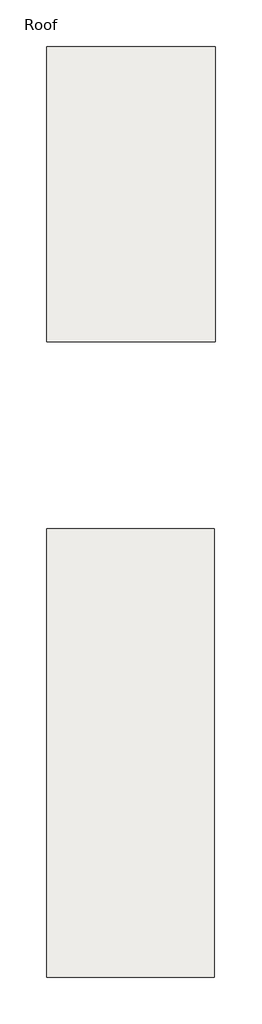
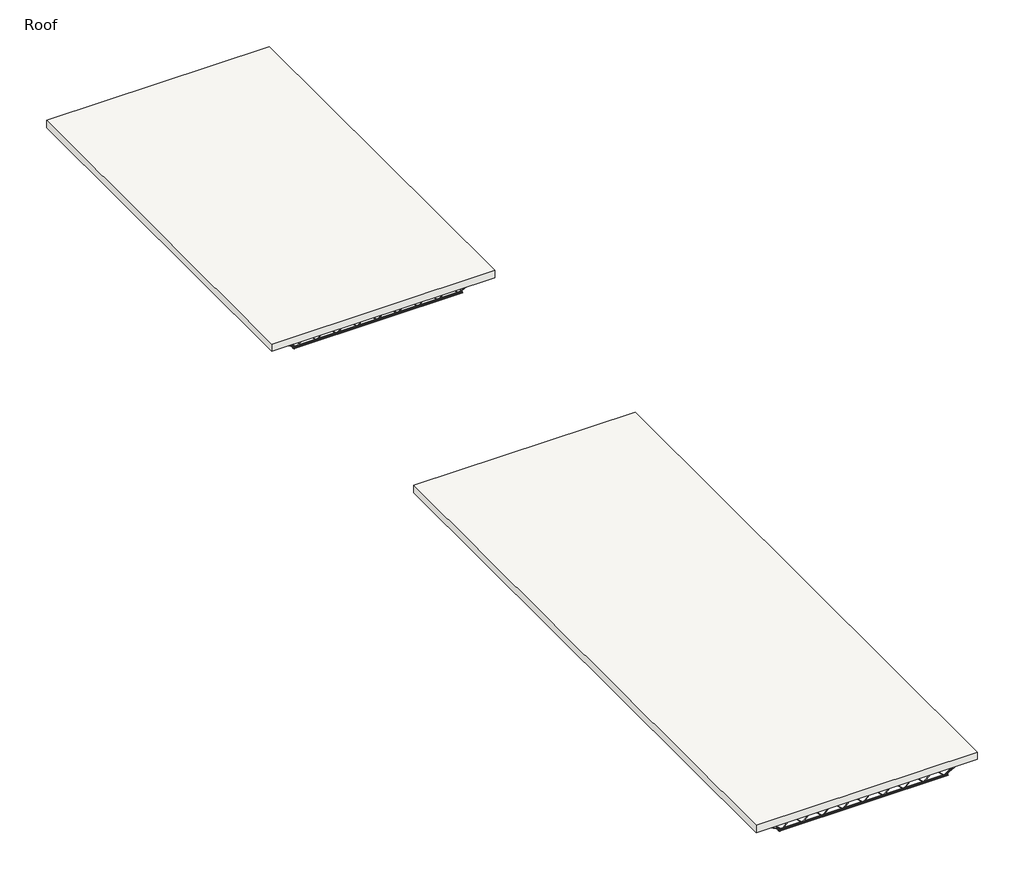
# One storey: 15 beams, 2 roofs.
"""IFC4 building model written with IfcOpenShell, lengths in millimetres."""

import ifcopenshell
import ifcopenshell.guid

model = None  # the IFC model being written
_history = None  # IfcOwnerHistory: only IFC2X3 demands one
_inside = {}  # id of a spatial element -> (the spatial element, [elements in it])
_under = {}  # id of a project, library or spatial element -> (it, [spatial elements below it])
_declared = {}  # id of a project -> (the project, [libraries it declares])
_typed = {}  # id of a type object -> (the type object, [elements of that type])
_made_of = {}  # id of a material, layer set ... -> (it, [elements and type objects made of it])


def new_model(schema):
    """Start an empty IFC model of exactly this schema.

    Asked for "IFC4X3", IfcOpenShell would pick the latest addendum, in which some entities
    have other attributes; the version numbers below select the first issue.
    IFC2X3 requires an IfcOwnerHistory on every rooted entity: one is made here for all.
    """
    global model, _history
    if schema == "IFC4X3":
        model = ifcopenshell.file(schema_version=(4, 3, 0, 0))
    else:
        model = ifcopenshell.file(schema=schema)
    _inside.clear()
    _under.clear()
    _declared.clear()
    _typed.clear()
    _made_of.clear()
    _history = None
    if model.schema == "IFC2X3":
        org = make("IfcOrganization", Name="unknown")
        user = make(
            "IfcPersonAndOrganization",
            ThePerson=make("IfcPerson", FamilyName="unknown"),
            TheOrganization=org,
        )
        app = make(
            "IfcApplication",
            ApplicationDeveloper=org,
            Version="unknown",
            ApplicationFullName="unknown",
            ApplicationIdentifier="unknown",
        )
        _history = make(
            "IfcOwnerHistory",
            OwningUser=user,
            OwningApplication=app,
            ChangeAction="ADDED",
            CreationDate=0,
        )
    return model


def make(cls, **values):
    """One entity of the class cls with the attributes given. An attribute that is None is left unset."""
    return model.create_entity(
        cls, **{name: value for name, value in values.items() if value is not None}
    )


def rooted(cls, **values):
    """An entity with a GlobalId (a new one), such as an element, a storey or a relation."""
    return make(cls, GlobalId=ifcopenshell.guid.new(), OwnerHistory=_history, **values)


def si_unit(unit_type, name, prefix=None):
    """IfcSIUnit, for example si_unit("LENGTHUNIT", "METRE", prefix="MILLI")."""
    return make("IfcSIUnit", UnitType=unit_type, Prefix=prefix, Name=name)


def assignment(units):
    """IfcUnitAssignment: the units of a project."""
    return None if units is None else make("IfcUnitAssignment", Units=units)


def point(xyz):
    """IfcCartesianPoint."""
    return None if xyz is None else make("IfcCartesianPoint", Coordinates=xyz)


def direction(xyz):
    """IfcDirection."""
    return None if xyz is None else make("IfcDirection", DirectionRatios=xyz)


def frame(location, z_axis=None, x_axis=None):
    """IfcAxis2Placement3D, a coordinate frame: its origin and axes. An axis left out is left unset."""
    return make(
        "IfcAxis2Placement3D",
        Location=point(location),
        Axis=direction(z_axis),
        RefDirection=direction(x_axis),
    )


def origin():
    """The frame at (0, 0, 0) with its axes left unset."""
    return frame((0.0, 0.0, 0.0))


def place(relative_to, where):
    """IfcLocalPlacement: puts the frame where relative to a parent placement (None: the world)."""
    return make(
        "IfcLocalPlacement", PlacementRelTo=relative_to, RelativePlacement=where
    )


def context(
    kind, dimensions, precision=None, world=None, true_north=None, identifier=None
):
    """IfcGeometricRepresentationContext, for example the 3D "Model" context."""
    return make(
        "IfcGeometricRepresentationContext",
        ContextIdentifier=identifier,
        ContextType=kind,
        CoordinateSpaceDimension=dimensions,
        Precision=precision,
        WorldCoordinateSystem=world,
        TrueNorth=true_north,
    )


def project(units=None, contexts=None):
    """IfcProject with its units and contexts."""
    return rooted(
        "IfcProject",
        Name="project",
        RepresentationContexts=contexts,
        UnitsInContext=assignment(units),
    )


def spatial(cls, under=None, at=None, **own):
    """A site, building, storey or space (cls), placed at a placement, below another one or the project."""
    s = rooted(cls, ObjectPlacement=at, **own)
    if under is not None:
        _under.setdefault(under.id(), (under, []))[1].append(s)
    return s


def polyline(points):
    """IfcPolyline through the points."""
    return make("IfcPolyline", Points=[point(p) for p in points])


def outline(outer, holes=None, kind="AREA"):
    """IfcArbitraryClosedProfileDef: a profile drawn as a closed curve; with holes, ...WithVoids."""
    if holes is None:
        return make("IfcArbitraryClosedProfileDef", ProfileType=kind, OuterCurve=outer)
    return make(
        "IfcArbitraryProfileDefWithVoids",
        ProfileType=kind,
        OuterCurve=outer,
        InnerCurves=holes,
    )


def extrude(swept, where, along, depth):
    """IfcExtrudedAreaSolid: the profile swept, set in the frame where, extruded along a direction by depth."""
    return make(
        "IfcExtrudedAreaSolid",
        SweptArea=swept,
        Position=where,
        ExtrudedDirection=direction(along),
        Depth=depth,
    )


def shape(context_of_items, identifier, shape_type, items):
    """IfcShapeRepresentation: the items that make up one representation, for example the "Body"."""
    return make(
        "IfcShapeRepresentation",
        ContextOfItems=context_of_items,
        RepresentationIdentifier=identifier,
        RepresentationType=shape_type,
        Items=items,
    )


def source(mapping_origin, context_of_items, identifier, shape_type, items):
    """IfcRepresentationMap: a shape defined once, which mapped items show again and again."""
    return make(
        "IfcRepresentationMap",
        MappingOrigin=mapping_origin,
        MappedRepresentation=shape(context_of_items, identifier, shape_type, items),
    )


def transform(
    local_origin,
    x_axis=None,
    y_axis=None,
    z_axis=None,
    scale=None,
    scale2=None,
    scale3=None,
    uniform=True,
):
    """IfcCartesianTransformationOperator3D, or its non-uniform kind. x_axis, y_axis, z_axis: its Axis1, 2, 3."""
    if uniform:
        return make(
            "IfcCartesianTransformationOperator3D",
            Axis1=direction(x_axis),
            Axis2=direction(y_axis),
            LocalOrigin=point(local_origin),
            Scale=scale,
            Axis3=direction(z_axis),
        )
    return make(
        "IfcCartesianTransformationOperator3DnonUniform",
        Axis1=direction(x_axis),
        Axis2=direction(y_axis),
        LocalOrigin=point(local_origin),
        Scale=scale,
        Axis3=direction(z_axis),
        Scale2=scale2,
        Scale3=scale3,
    )


def mapped(mapping_source, mapping_target):
    """IfcMappedItem: shows the shape of a source again, moved by a transform."""
    return make(
        "IfcMappedItem", MappingSource=mapping_source, MappingTarget=mapping_target
    )


def made_of(thing, what):
    """Note that an element or type object is made of a material, layer set ...; save() writes the relation."""
    if what is not None:
        _made_of.setdefault(what.id(), (what, []))[1].append(thing)
    return thing


def element(
    cls,
    number,
    at=None,
    inside=None,
    cuts=None,
    type_object=None,
    material=None,
    context=None,
    identifier="Body",
    shape_type=None,
    held_by="IfcProductDefinitionShape",
    body=None,
    shapes=None,
    **own,
):
    """One element of the class cls, such as IfcWall. Its Tag is "e" and its number.

    at: its placement. inside: the storey or other place that contains it. cuts: it is an
    opening in that element (IfcRelVoidsElement). A single representation is given by context,
    identifier, shape_type and body (its items); several are given by shapes. held_by: the class
    of the entity that holds the representations. save() writes the other relations.
    """
    e = rooted(cls, Tag="e%d" % number, ObjectPlacement=at, **own)
    if body is not None:
        shapes = [shape(context, identifier, shape_type, body)]
    if shapes is not None:
        e.Representation = make(held_by, Representations=shapes)
    if inside is not None:
        _inside.setdefault(inside.id(), (inside, []))[1].append(e)
    if cuts is not None:
        rooted(
            "IfcRelVoidsElement", RelatingBuildingElement=cuts, RelatedOpeningElement=e
        )
    if type_object is not None:
        _typed.setdefault(type_object.id(), (type_object, []))[1].append(e)
    return made_of(e, material)


def aggregate(whole, parts):
    """IfcRelAggregates: a whole, such as a stair, and the parts it consists of."""
    return rooted("IfcRelAggregates", RelatingObject=whole, RelatedObjects=parts)


def save(model, path):
    """Write the relations noted so far, then the file.

    IfcRelAggregates (storeys below a building ...), IfcRelContainedInSpatialStructure (elements
    in a storey), IfcRelDefinesByType, IfcRelAssociatesMaterial and IfcRelDeclares: one each for
    every whole, place, type object, material and project.
    """
    for whole, parts in _under.values():
        aggregate(whole, parts)
    for where, things in _inside.values():
        rooted(
            "IfcRelContainedInSpatialStructure",
            RelatedElements=things,
            RelatingStructure=where,
        )
    for kind, things in _typed.values():
        rooted("IfcRelDefinesByType", RelatedObjects=things, RelatingType=kind)
    for what, things in _made_of.values():
        rooted("IfcRelAssociatesMaterial", RelatedObjects=things, RelatingMaterial=what)
    for by, libraries in _declared.values():
        rooted("IfcRelDeclares", RelatingContext=by, RelatedDefinitions=libraries)
    model.write(path)


def k_series_bar_joist_rod_web_12k5_aa514e25(model_context):
    return source(origin(), model_context, "Body", "SweptSolid", [
        extrude(outline(polyline([(-141.2875, 1209.1080357), (-150.8125, 1209.1080357), (-150.8125, 1214.2369297), (141.2875, 1510.3056797), (141.2875, 1512.7478918), (-150.8125, 1808.8166418), (-150.8125, 1813.9455357), (-141.2875, 1813.9455357), (-141.2875, 1812.7244297), (150.8125, 1516.6556797), (150.8125, 1506.3978918), (-141.2875, 1210.3291418), (-141.2875, 1209.1080357)])), frame((0.0, -4.7625, 0.0), z_axis=(0.0, 1.0, 0.0), x_axis=(0.0, 0.0, 1.0)), (0.0, 0.0, 1.0), 9.525),
        extrude(outline(polyline([(-141.2875, 604.4973214), (-150.8125, 604.4973214), (-150.8125, 609.6262154), (141.2875, 905.6949654), (141.2875, 908.1371775), (-150.8125, 1204.2059275), (-150.8125, 1209.3348214), (-141.2875, 1209.3348214), (-141.2875, 1208.1137154), (150.8125, 912.0449654), (150.8125, 901.7871775), (-141.2875, 605.7184275), (-141.2875, 604.4973214)])), frame((0.0, -4.7625, 0.0), z_axis=(0.0, 1.0, 0.0), x_axis=(0.0, 0.0, 1.0)), (0.0, 0.0, 1.0), 9.525),
        extrude(outline(polyline([(-141.2875, -0.1133929), (-150.8125, -0.1133929), (-150.8125, 5.0155011), (141.2875, 301.0842511), (141.2875, 303.5264632), (-150.8125, 599.5952132), (-150.8125, 604.7241071), (-141.2875, 604.7241071), (-141.2875, 603.5030011), (150.8125, 307.4342511), (150.8125, 297.1764632), (-141.2875, 1.1077132), (-141.2875, -0.1133929)])), frame((0.0, -4.7625, 0.0), z_axis=(0.0, 1.0, 0.0), x_axis=(0.0, 0.0, 1.0)), (0.0, 0.0, 1.0), 9.525),
        extrude(outline(polyline([(-141.2875, -604.7241071), (-150.8125, -604.7241071), (-150.8125, -599.5952132), (141.2875, -303.5264632), (141.2875, -301.0842511), (-150.8125, -5.0155011), (-150.8125, 0.1133929), (-141.2875, 0.1133929), (-141.2875, -1.1077132), (150.8125, -297.1764632), (150.8125, -307.4342511), (-141.2875, -603.5030011), (-141.2875, -604.7241071)])), frame((0.0, -4.7625, 0.0), z_axis=(0.0, 1.0, 0.0), x_axis=(0.0, 0.0, 1.0)), (0.0, 0.0, 1.0), 9.525),
        extrude(outline(polyline([(-141.2875, -1209.3348214), (-150.8125, -1209.3348214), (-150.8125, -1204.2059275), (141.2875, -908.1371775), (141.2875, -905.6949654), (-150.8125, -609.6262154), (-150.8125, -604.4973214), (-141.2875, -604.4973214), (-141.2875, -605.7184275), (150.8125, -901.7871775), (150.8125, -912.0449654), (-141.2875, -1208.1137154), (-141.2875, -1209.3348214)])), frame((0.0, -4.7625, 0.0), z_axis=(0.0, 1.0, 0.0), x_axis=(0.0, 0.0, 1.0)), (0.0, 0.0, 1.0), 9.525),
        extrude(outline(polyline([(-141.2875, -1813.9455357), (-150.8125, -1813.9455357), (-150.8125, -1808.8166418), (141.2875, -1512.7478918), (141.2875, -1510.3056797), (-150.8125, -1214.2369297), (-150.8125, -1209.1080357), (-141.2875, -1209.1080357), (-141.2875, -1210.3291418), (150.8125, -1506.3978918), (150.8125, -1516.6556797), (-141.2875, -1812.7244297), (-141.2875, -1813.9455357)])), frame((0.0, -4.7625, 0.0), z_axis=(0.0, 1.0, 0.0), x_axis=(0.0, 0.0, 1.0)), (0.0, 0.0, 1.0), 9.525),
        extrude(outline(polyline([(-141.2875, 1813.71875), (-150.8125, 1813.71875), (-150.8125, 1818.847644), (141.2875, 2114.916394), (141.2875, 2117.358606), (-150.8125, 2413.427356), (-150.8125, 2418.55625), (-141.2875, 2418.55625), (-141.2875, 2417.335144), (150.8125, 2121.266394), (150.8125, 2111.008606), (-141.2875, 1814.939856), (-141.2875, 1813.71875)])), frame((0.0, -4.7625, 0.0), z_axis=(0.0, 1.0, 0.0), x_axis=(0.0, 0.0, 1.0)), (0.0, 0.0, 1.0), 9.525),
        extrude(outline(polyline([(-141.2875, -2418.55625), (-150.8125, -2418.55625), (-150.8125, -2413.427356), (141.2875, -2117.358606), (141.2875, -2114.916394), (-150.8125, -1818.847644), (-150.8125, -1813.71875), (-141.2875, -1813.71875), (-141.2875, -1814.939856), (150.8125, -2111.008606), (150.8125, -2121.266394), (-141.2875, -2417.335144), (-141.2875, -2418.55625)])), frame((0.0, -4.7625, 0.0), z_axis=(0.0, 1.0, 0.0), x_axis=(0.0, 0.0, 1.0)), (0.0, 0.0, 1.0), 9.525),
        extrude(outline(polyline([(4.7625, 152.4), (36.5125, 152.4), (36.5125, 146.05), (11.1125, 146.05), (11.1125, 120.65), (4.7625, 120.65), (4.7625, 152.4)])), frame((-3028.15625, 0.0, 0.0), z_axis=(1.0, 0.0, 0.0), x_axis=(0.0, 1.0, 0.0)), (0.0, 0.0, 1.0), 6056.3125),
        extrude(outline(polyline([(-4.7625, 152.4), (-4.7625, 120.65), (-11.1125, 120.65), (-11.1125, 146.05), (-36.5125, 146.05), (-36.5125, 152.4), (-4.7625, 152.4)])), frame((-3028.15625, 0.0, 0.0), z_axis=(1.0, 0.0, 0.0), x_axis=(0.0, 1.0, 0.0)), (0.0, 0.0, 1.0), 6056.3125),
        extrude(outline(polyline([(-4.7625, 88.9), (-36.5125, 88.9), (-36.5125, 95.25), (-11.1125, 95.25), (-11.1125, 120.65), (-4.7625, 120.65), (-4.7625, 88.9)])), frame((-3028.15625, 0.0, 0.0), z_axis=(1.0, 0.0, 0.0), x_axis=(0.0, 1.0, 0.0)), (0.0, 0.0, 1.0), 101.6),
        extrude(outline(polyline([(36.5125, 88.9), (4.7625, 88.9), (4.7625, 120.65), (11.1125, 120.65), (11.1125, 95.25), (36.5125, 95.25), (36.5125, 88.9)])), frame((-3028.15625, 0.0, 0.0), z_axis=(1.0, 0.0, 0.0), x_axis=(0.0, 1.0, 0.0)), (0.0, 0.0, 1.0), 101.6),
        extrude(outline(polyline([(4.7625, 88.9), (4.7625, 120.65), (11.1125, 120.65), (11.1125, 95.25), (36.5125, 95.25), (36.5125, 88.9), (4.7625, 88.9)])), frame((2926.55625, 0.0, 0.0), z_axis=(1.0, 0.0, 0.0), x_axis=(0.0, 1.0, 0.0)), (0.0, 0.0, 1.0), 101.6),
        extrude(outline(polyline([(-4.7625, 88.9), (-36.5125, 88.9), (-36.5125, 95.25), (-11.1125, 95.25), (-11.1125, 120.65), (-4.7625, 120.65), (-4.7625, 88.9)])), frame((2926.55625, 0.0, 0.0), z_axis=(1.0, 0.0, 0.0), x_axis=(0.0, 1.0, 0.0)), (0.0, 0.0, 1.0), 101.6),
        extrude(outline(polyline([(4.7625, -152.4), (4.7625, -120.65), (11.1125, -120.65), (11.1125, -146.05), (36.5125, -146.05), (36.5125, -152.4), (4.7625, -152.4)])), frame((-2520.15625, 0.0, 0.0), z_axis=(1.0, 0.0, 0.0), x_axis=(0.0, 1.0, 0.0)), (0.0, 0.0, 1.0), 5040.3125),
        extrude(outline(polyline([(-4.7625, -152.4), (-36.5125, -152.4), (-36.5125, -146.05), (-11.1125, -146.05), (-11.1125, -120.65), (-4.7625, -120.65), (-4.7625, -152.4)])), frame((-2520.15625, 0.0, 0.0), z_axis=(1.0, 0.0, 0.0), x_axis=(0.0, 1.0, 0.0)), (0.0, 0.0, 1.0), 5040.3125),
        extrude(outline(polyline([(0.0, -9.525), (0.0, 0.0), (573.7533355, 0.0), (573.7533355, -9.525), (0.0, -9.525)])), frame((-2928.7700214, 4.7625, 116.4332925), z_axis=(0.4648338989895367, 0.0, 0.885397902838145), x_axis=(0.885397902838145, 0.0, -0.4648338989895367)), (0.0, 0.0, 1.0), 9.525),
        extrude(outline(polyline([(0.0, -9.525), (0.0, 0.0), (403.2195312, 0.0), (403.2195312, -9.525), (0.0, -9.525)])), frame((-2724.1250427, 4.7625, 117.0780766), z_axis=(0.6614262935071406, 0.0, 0.750010172102623), x_axis=(0.750010172102623, 0.0, -0.6614262935071406)), (0.0, 0.0, 1.0), 9.525),
        extrude(outline(polyline([(0.0, -9.525), (0.0, 0.0), (573.7533355, 0.0), (573.7533355, -9.525), (0.0, -9.525)])), frame((2928.7700214, -4.7625, 116.4332925), z_axis=(-0.4648338989895162, 0.0, 0.8853979028381558), x_axis=(-0.8853979028381558, 0.0, -0.4648338989895162)), (0.0, 0.0, 1.0), 9.525),
        extrude(outline(polyline([(0.0, -9.525), (0.0, 0.0), (403.2195312, 0.0), (403.2195312, -9.525), (0.0, -9.525)])), frame((2724.1250427, -4.7625, 117.0780766), z_axis=(-0.6614262935071337, 0.0, 0.7500101721026291), x_axis=(-0.7500101721026291, 0.0, -0.6614262935071337)), (0.0, 0.0, 1.0), 9.525),
    ])


model = new_model("IFC4")

# Units and contexts
model_context = context("Model", 3, world=origin())
ifc_project = project(units=[si_unit("LENGTHUNIT", "METRE", prefix="MILLI")], contexts=[model_context])

# Site, building, storey
site = spatial("IfcSite", under=ifc_project)
building = spatial("IfcBuilding", under=site)
storey = spatial("IfcBuildingStorey", under=building, Name="Roof", Elevation=7315.2)

# Beams
placement = place(None, origin())
k_series_bar_joist_rod_web_12k5_shape = k_series_bar_joist_rod_web_12k5_aa514e25(model_context)
element("IfcBeam", 1, ObjectType="K-Series Bar Joist-Rod Web : 12K5", at=placement, inside=storey, context=model_context, shape_type="MappedRepresentation", body=[
    mapped(k_series_bar_joist_rod_web_12k5_shape, transform((-3185.7901664, -613.4201131, 7162.8), x_axis=(-1.0, 0.0, 0.0), y_axis=(0.0, -1.0, 0.0), z_axis=(0.0, 0.0, 1.0))),
])
element("IfcBeam", 2, ObjectType="K-Series Bar Joist-Rod Web : 12K5", at=placement, inside=storey, context=model_context, shape_type="MappedRepresentation", body=[
    mapped(k_series_bar_joist_rod_web_12k5_shape, transform((-3185.7901664, 1554.6513154, 7162.8), x_axis=(-1.0, 0.0, 0.0), y_axis=(0.0, -1.0, 0.0), z_axis=(0.0, 0.0, 1.0))),
])
element("IfcBeam", 3, ObjectType="K-Series Bar Joist-Rod Web : 12K5", at=placement, inside=storey, context=model_context, shape_type="MappedRepresentation", body=[
    mapped(k_series_bar_joist_rod_web_12k5_shape, transform((-3185.7901664, 3722.722744, 7162.8), x_axis=(-1.0, 0.0, 0.0), y_axis=(0.0, -1.0, 0.0), z_axis=(0.0, 0.0, 1.0))),
])
element("IfcBeam", 4, ObjectType="K-Series Bar Joist-Rod Web : 12K5", at=placement, inside=storey, context=model_context, shape_type="MappedRepresentation", body=[
    mapped(k_series_bar_joist_rod_web_12k5_shape, transform((-3185.7901664, 5890.7941726, 7162.8), x_axis=(-1.0, 0.0, 0.0), y_axis=(0.0, -1.0, 0.0), z_axis=(0.0, 0.0, 1.0))),
])
element("IfcBeam", 5, ObjectType="K-Series Bar Joist-Rod Web : 12K5", at=placement, inside=storey, context=model_context, shape_type="MappedRepresentation", body=[
    mapped(k_series_bar_joist_rod_web_12k5_shape, transform((-3185.7901664, 8058.8656011, 7162.8), x_axis=(-1.0, 0.0, 0.0), y_axis=(0.0, -1.0, 0.0), z_axis=(0.0, 0.0, 1.0))),
])
element("IfcBeam", 6, ObjectType="K-Series Bar Joist-Rod Web : 12K5", at=placement, inside=storey, context=model_context, shape_type="MappedRepresentation", body=[
    mapped(k_series_bar_joist_rod_web_12k5_shape, transform((-3185.7901664, 10226.9370297, 7162.8), x_axis=(-1.0, 0.0, 0.0), y_axis=(0.0, -1.0, 0.0), z_axis=(0.0, 0.0, 1.0))),
])
element("IfcBeam", 7, ObjectType="K-Series Bar Joist-Rod Web : 12K5", at=placement, inside=storey, context=model_context, shape_type="MappedRepresentation", body=[
    mapped(k_series_bar_joist_rod_web_12k5_shape, transform((-3185.7901664, 12395.0084583, 7162.8), x_axis=(-1.0, 0.0, 0.0), y_axis=(0.0, -1.0, 0.0), z_axis=(0.0, 0.0, 1.0))),
])
element("IfcBeam", 8, ObjectType="K-Series Bar Joist-Rod Web : 12K5", at=placement, inside=storey, context=model_context, shape_type="MappedRepresentation", body=[
    mapped(k_series_bar_joist_rod_web_12k5_shape, transform((-3185.7901664, 14563.0798869, 7162.8), x_axis=(-1.0, 0.0, 0.0), y_axis=(0.0, -1.0, 0.0), z_axis=(0.0, 0.0, 1.0))),
])
element("IfcBeam", 9, ObjectType="K-Series Bar Joist-Rod Web : 12K5", at=placement, inside=storey, context=model_context, shape_type="MappedRepresentation", body=[
    mapped(k_series_bar_joist_rod_web_12k5_shape, transform((-3185.7901664, 16731.1513154, 7162.8), x_axis=(-1.0, 0.0, 0.0), y_axis=(0.0, -1.0, 0.0), z_axis=(0.0, 0.0, 1.0))),
])
element("IfcBeam", 10, ObjectType="K-Series Bar Joist-Rod Web : 12K5", at=placement, inside=storey, context=model_context, shape_type="MappedRepresentation", body=[
    mapped(k_series_bar_joist_rod_web_12k5_shape, transform((-3185.7901664, 24446.4013154, 7162.8), x_axis=(-1.0, 0.0, 0.0), y_axis=(0.0, -1.0, 0.0), z_axis=(0.0, 0.0, 1.0))),
])
element("IfcBeam", 11, ObjectType="K-Series Bar Joist-Rod Web : 12K5", at=placement, inside=storey, context=model_context, shape_type="MappedRepresentation", body=[
    mapped(k_series_bar_joist_rod_web_12k5_shape, transform((-3185.7901664, 35609.7013154, 7162.8), x_axis=(-1.0, 0.0, 0.0), y_axis=(0.0, -1.0, 0.0), z_axis=(0.0, 0.0, 1.0))),
])
element("IfcBeam", 12, ObjectType="K-Series Bar Joist-Rod Web : 12K5", at=placement, inside=storey, context=model_context, shape_type="MappedRepresentation", body=[
    mapped(k_series_bar_joist_rod_web_12k5_shape, transform((-3185.7901664, 26679.0613154, 7162.8), x_axis=(-1.0, 0.0, 0.0), y_axis=(0.0, -1.0, 0.0), z_axis=(0.0, 0.0, 1.0))),
])
element("IfcBeam", 13, ObjectType="K-Series Bar Joist-Rod Web : 12K5", at=placement, inside=storey, context=model_context, shape_type="MappedRepresentation", body=[
    mapped(k_series_bar_joist_rod_web_12k5_shape, transform((-3185.7901664, 28911.7213154, 7162.8), x_axis=(-1.0, 0.0, 0.0), y_axis=(0.0, -1.0, 0.0), z_axis=(0.0, 0.0, 1.0))),
])
element("IfcBeam", 14, ObjectType="K-Series Bar Joist-Rod Web : 12K5", at=placement, inside=storey, context=model_context, shape_type="MappedRepresentation", body=[
    mapped(k_series_bar_joist_rod_web_12k5_shape, transform((-3185.7901664, 31144.3813154, 7162.8), x_axis=(-1.0, 0.0, 0.0), y_axis=(0.0, -1.0, 0.0), z_axis=(0.0, 0.0, 1.0))),
])
element("IfcBeam", 15, ObjectType="K-Series Bar Joist-Rod Web : 12K5", at=placement, inside=storey, context=model_context, shape_type="MappedRepresentation", body=[
    mapped(k_series_bar_joist_rod_web_12k5_shape, transform((-3185.7901664, 33377.0413154, 7162.8), x_axis=(-1.0, 0.0, 0.0), y_axis=(0.0, -1.0, 0.0), z_axis=(0.0, 0.0, 1.0))),
])

# Roofs
element("IfcRoof", 16, ObjectType="9\" - Corrugated Deck + Insulation", at=placement, inside=storey, context=model_context, shape_type="SweptSolid", body=[
    extrude(outline(polyline([(-6468.7401664, -782.1486846), (-6468.7401664, 16878.1084583), (122.5598336, 16878.1084583), (122.5598336, -782.1486846), (-6468.7401664, -782.1486846)])), frame((0.0, 0.0, 7315.2), z_axis=(0.0, 0.0, 1.0), x_axis=(1.0, 0.0, 0.0)), (0.0, 0.0, 1.0), 228.6),
])
element("IfcRoof", 17, ObjectType="9\" - Corrugated Deck + Insulation", at=placement, inside=storey, context=model_context, shape_type="SweptSolid", body=[
    extrude(outline(polyline([(-6468.7401664, 24217.8013154), (-6468.7401664, 35838.3013154), (173.3598336, 35838.3013154), (173.3598336, 24217.8013154), (-6468.7401664, 24217.8013154)])), frame((0.0, 0.0, 7315.2), z_axis=(0.0, 0.0, 1.0), x_axis=(1.0, 0.0, 0.0)), (0.0, 0.0, 1.0), 228.6),
])

save(model, "model.ifc")

# Revit data of these elements
# Project information
#   SR Document GUID = "7e8cea01-ee78-400c-8c48-bf15b658b500"
# Type "K-Series Bar Joist-Rod Web : 12K5"
#   Assembly Code = "B1010350"
#   Wt = 7.1
#   Web Thickness = 9.525 mm
#   Start Offset [instance default] = 0.00 mm
#   Start Extension [instance default] = 0.00 mm
#   Seat Length = 101.60 mm
#   Seat Depth = 63.50 mm
#   PanelArrayLength [instance default] = 6096.00 mm
#   Panel [instance default] = 609.60 mm
#   End Offset [instance default] = 0.00 mm
#   End Extension [instance default] = 0.00 mm
#   End Panel = 609.60 mm
#   Cord Leg = 31.75 mm
#   Chord Thickness = 6.35 mm
#   Length [instance default] = 7315.20 mm
#   Depth = 304.80 mm
#   PanelArrayNum [instance default] = 10
#   Structural Material = none
# Type "9\" - Corrugated Deck + Insulation"
#   built-in parameter 1001600 = 0.75 (stored number, unit not read)
#   Layers, outside or top first: 12.70 mm "Roofing - Generic" (function 4); 139.70 mm "Insulation / Thermal Barriers - Rigid insulation" (function 3); 76.20 mm "Metal - Deck" (function 1)
# Elements 1, 2, 3, 4, 5, 6, 7, 8, 9, 10, 11, 12, 13, 14, 15 (IfcBeam, "K-Series Bar Joist-Rod Web : 12K5")
#   Start Offset = 0.00 mm
#   Start Extension = 0.00 mm
#   PanelArrayLength = 4838.70 mm
#   Panel = 604.837 mm
#   End Offset = 0.00 mm
#   End Extension = 0.00 mm
#   PanelArrayNum = 8
#   Phase Created = New Construction
# Elements 16, 17 (IfcRoof, "9\" - Corrugated Deck + Insulation")
#   built-in parameter 1001705 = 24.75 (stored number, unit not read)
#   built-in parameter 1001710 = 33615
#   Phase Created = New Construction
#   Materials on its faces: "Metal - Deck", "Roofing - Generic"
# Materials
#   "Roofing - Generic": class "Paint", colour RGB 138 138 138, transparency 0, Description = "Exterior finish, roofing"
#   "Insulation / Thermal Barriers - Rigid insulation": class "Miscellaneous", colour RGB 219 205 164, transparency 0
#   "Metal - Deck": class "Metal", colour RGB 199 199 199, transparency 0
